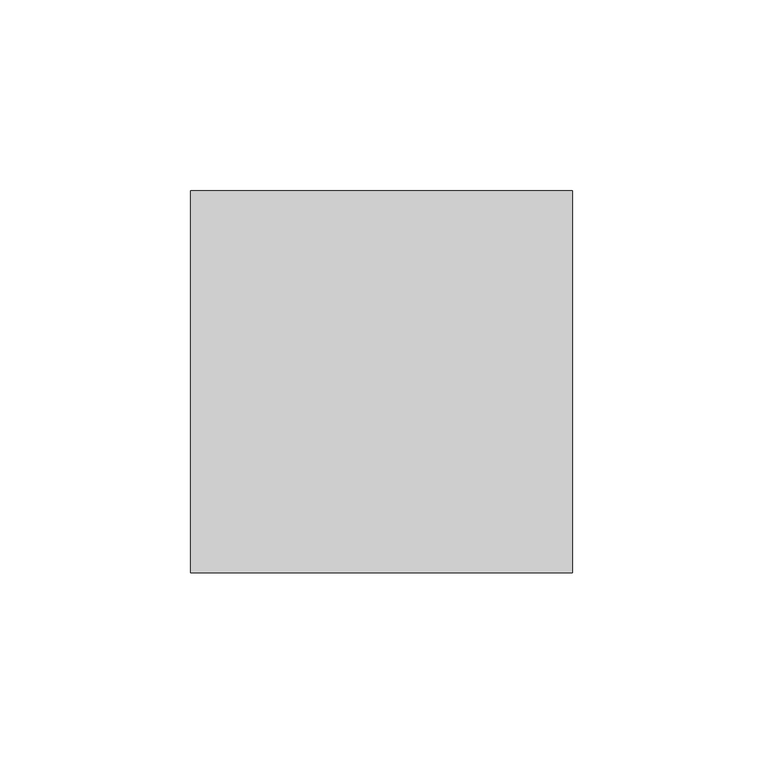
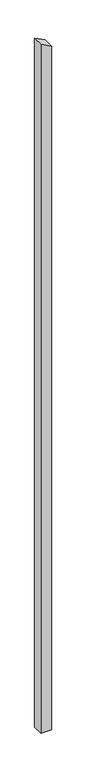
"""IFC4 building model written with IfcOpenShell, lengths in millimetres: column geometry, Holzstütze 159106 : Holzstütze 159106."""

from ifc_helpers import new_model, si_unit, frame, origin, place, context, project, spatial, polyline, outline, extrude, source, transform, mapped, element, save


def column_a4466fb5(model_context):
    return source(origin(), model_context, "Body", "SweptSolid", [
        extrude(outline(polyline([(-500.0, 174197.7593015), (-500.0, 174297.7593015), (6345.7118258, 174297.7593015), (6396.6643707, 174197.7593015), (-500.0, 174197.7593015)])), frame((0.0, 31941.5369795, 0.0), z_axis=(0.0, 1.0, 0.0), x_axis=(0.0, 0.0, 1.0)), (0.0, 0.0, 1.0), 100.0),
    ])


if __name__ == "__main__":
    model = new_model("IFC4")
    model_context = context("Model", 3, world=origin())
    ifc_project = project(units=[si_unit("LENGTHUNIT", "METRE", prefix="MILLI")], contexts=[model_context])
    site = spatial("IfcSite", under=ifc_project)
    building = spatial("IfcBuilding", under=site)
    placement = place(None, origin())
    column_shape = column_a4466fb5(model_context)
    element("IfcColumn", 1, ObjectType="Holzstütze 159106 : Holzstütze 159106", at=placement, inside=building, context=model_context, shape_type="MappedRepresentation", body=[
        mapped(column_shape, transform((0.0, 0.0, 0.0), x_axis=(1.0, 0.0, 0.0), y_axis=(0.0, 1.0, 0.0), z_axis=(0.0, 0.0, 1.0))),
    ])
    save(model, "model.ifc")

# Revit data of these elements
# Type "Holzstütze 159106 : Holzstütze 159106"
#   Abrechnungsart = "m"
#   Allright_Bauteil_ID = "0152St 0000143487"
#   Bezeichnung = "Holzstütze"
#   Codetext = "ST-HOLZ\\"
#   Gewerk = "Zimmer- und Holzbauarbeiten"
#   Material = "Holz"
#   Objektname = "Stütze"
#   NameOverride = "Holzstütze"
#   Reference = "Holzstütze"
#   Status = "NEW"
#   ThermalTransmittance = 0.0000 BTU/(h·ft²·°F)
#   Roll = 0.00°
#   Slope = 0.00°
#   2D Interaktion = yes
#   IsExternal = yes
#   LoadBearing = yes
# Element 1 (IfcColumn, "Holzstütze 159106 : Holzstütze 159106")
#   Materials on its faces: "holzschalung"
# Materials
#   "holzschalung": class "Unassigned", colour RGB 128 128 128, transparency 0
